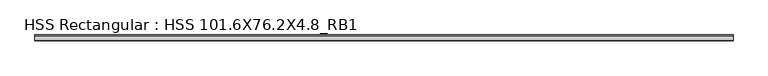
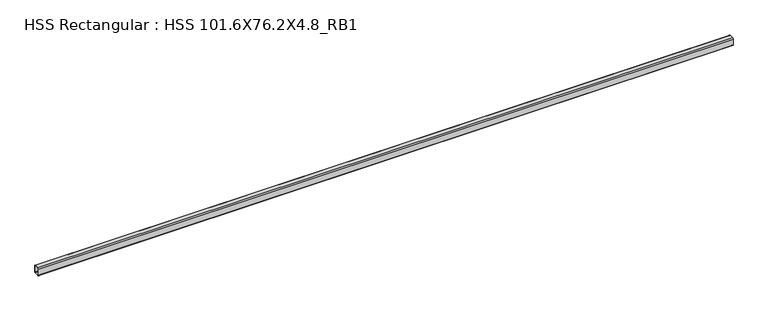
"""IFC4 building model written with IfcOpenShell, lengths in millimetres: beam geometry, HSS Rectangular : HSS 101.6X76.2X4.8_RB1."""

from ifc_helpers import new_model, si_unit, point, frame, frame_2d, origin, place, context, project, spatial, polyline, circle_curve, trimmed, segment, composite_curve, outline, extrude, source, transform, mapped, element, save


def hss_rectangular_hss_101_6x76_2x4_8_rb1_eb83d95e(model_context):
    return source(origin(), model_context, "Body", "SweptSolid", [
        extrude(outline(composite_curve([segment(polyline([(38.1, 41.275), (38.1, -41.275)]), True, "CONTINUOUS"), segment(trimmed(circle_curve(frame_2d((28.575, -41.275)), 9.525), [point((38.1, -41.275))], [point((28.575, -50.8))], False, "CARTESIAN"), True, "CONTINUOUS"), segment(polyline([(28.575, -50.8), (-28.575, -50.8)]), True, "CONTINUOUS"), segment(trimmed(circle_curve(frame_2d((-28.575, -41.275)), 9.525), [point((-28.575, -50.8))], [point((-38.1, -41.275))], False, "CARTESIAN"), True, "CONTINUOUS"), segment(polyline([(-38.1, -41.275), (-38.1, 41.275)]), True, "CONTINUOUS"), segment(trimmed(circle_curve(frame_2d((-28.575, 41.275)), 9.525), [point((-38.1, 41.275))], [point((-28.575, 50.8))], False, "CARTESIAN"), True, "CONTINUOUS"), segment(polyline([(-28.575, 50.8), (28.575, 50.8)]), True, "CONTINUOUS"), segment(trimmed(circle_curve(frame_2d((28.575, 41.275)), 9.525), [point((28.575, 50.8))], [point((38.1, 41.275))], False, "CARTESIAN"), True, "CONTINUOUS")], self_intersect=False), holes=[composite_curve([segment(trimmed(circle_curve(frame_2d((-28.575, 41.275)), 4.7625), [point((-28.575, 46.0375))], [point((-33.3375, 41.275))], True, "CARTESIAN"), True, "CONTINUOUS"), segment(polyline([(-33.3375, 41.275), (-33.3375, -41.275)]), True, "CONTINUOUS"), segment(trimmed(circle_curve(frame_2d((-28.575, -41.275)), 4.7625), [point((-33.3375, -41.275))], [point((-28.575, -46.0375))], True, "CARTESIAN"), True, "CONTINUOUS"), segment(polyline([(-28.575, -46.0375), (28.575, -46.0375)]), True, "CONTINUOUS"), segment(trimmed(circle_curve(frame_2d((28.575, -41.275)), 4.7625), [point((28.575, -46.0375))], [point((33.3375, -41.275))], True, "CARTESIAN"), True, "CONTINUOUS"), segment(polyline([(33.3375, -41.275), (33.3375, 41.275)]), True, "CONTINUOUS"), segment(trimmed(circle_curve(frame_2d((28.575, 41.275)), 4.7625), [point((33.3375, 41.275))], [point((28.575, 46.0375))], True, "CARTESIAN"), True, "CONTINUOUS"), segment(polyline([(28.575, 46.0375), (-28.575, 46.0375)]), True, "CONTINUOUS")], self_intersect=False)]), frame((-10554.478596, 0.0, 0.0), z_axis=(1.0, 0.0, 0.0), x_axis=(0.0, 1.0, 0.0)), (0.0, 0.0, 1.0), 8925.0508079),
    ])


if __name__ == "__main__":
    model = new_model("IFC4")
    model_context = context("Model", 3, world=origin())
    ifc_project = project(units=[si_unit("LENGTHUNIT", "METRE", prefix="MILLI")], contexts=[model_context])
    site = spatial("IfcSite", under=ifc_project)
    building = spatial("IfcBuilding", under=site)
    placement = place(None, origin())
    hss_rectangular_hss_101_6x76_2x4_8_rb1_shape = hss_rectangular_hss_101_6x76_2x4_8_rb1_eb83d95e(model_context)
    element("IfcBeam", 1, ObjectType="HSS Rectangular : HSS 101.6X76.2X4.8_RB1", at=placement, inside=building, context=model_context, shape_type="MappedRepresentation", body=[
        mapped(hss_rectangular_hss_101_6x76_2x4_8_rb1_shape, transform((0.0, 0.0, 0.0), x_axis=(1.0, 0.0, 0.0), y_axis=(0.0, 1.0, 0.0), z_axis=(0.0, 0.0, 1.0))),
    ])
    save(model, "model.ifc")

# Revit data of these elements
# Type "HSS Rectangular : HSS 101.6X76.2X4.8_RB1"
#   Section Name Key = "HSS 4X3X3/16"
#   Assembly Code = "B10"
#   Width = 7.62 cm
#   Wall Nominal Thickness = 0.4763 cm
#   Wall Design Thickness = 0.442 cm
#   Torsional Moment of Inertia = 260.561 cm⁴
#   Torsional Modulus = 61.2876 cm³
#   Section Area = 14.4516 cm²
#   Plastic Modulus weak axis = 40.3122 cm³
#   Plastic Modulus strong axis = 49.1612 cm³
#   Perimeter = 0.881482 m²/m
#   Outer Fillet = 0.9525 cm
#   Nominal Weight = 12.1285 kgf/m
#   Moment of Inertia weak axis = 131.529 cm⁴
#   Moment of Inertia strong axis = 205.202 cm⁴
#   Inner Fillet = 0.4763 cm
#   Height = 10.16 cm
#   Elastic Modulus weak axis = 34.4128 cm³
#   Elastic Modulus strong axis = 40.476 cm³
#   Centroid Vertical = 5.08 cm
#   Centroid Horizontal = 3.81 cm
#   Length [instance default] = 1524 mm
#   Structural Material [instance default] = Steel ASTM A500, Grade B, Rectangular and Square
#   Principal Axes Angle = 0
# Element 1 (IfcBeam, "HSS Rectangular : HSS 101.6X76.2X4.8_RB1")
#   Structural Material = Steel ASTM A992
#   Materials on its faces: "Steel ASTM A992"
# Materials
#   "Steel ASTM A500, Grade B, Rectangular and Square": class "Metal", colour RGB 199 199 199, transparency 0, Description = "Carbon steel", Cost = 0
#   "Steel ASTM A992": class "Metal", colour RGB 199 199 199, transparency 0, Description = "Structural steel 50ksi", Cost = 0
